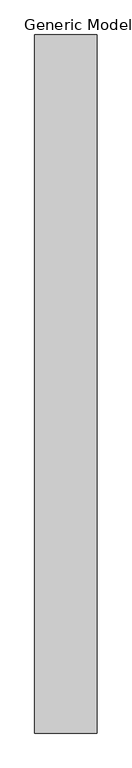
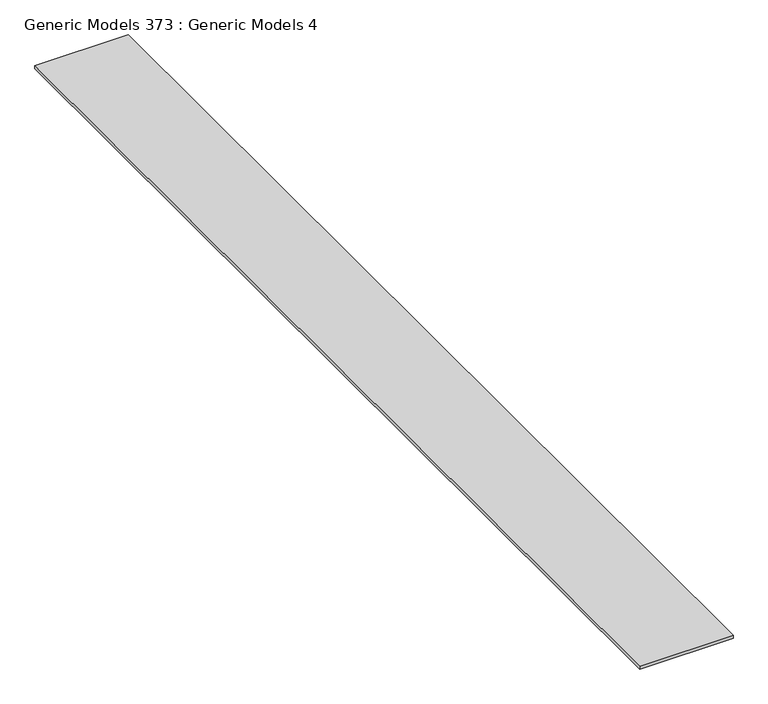
"""IFC4 building model written with IfcOpenShell, lengths in millimetres: proxy geometry, Generic Models 373 : Generic Models 4."""

from ifc_helpers import new_model, si_unit, frame, origin, place, context, project, spatial, polyline, outline, extrude, source, transform, mapped, element, save


def generic_models_373_generic_models_4_3e0b37f2(model_context):
    return source(origin(), model_context, "Body", "SweptSolid", [
        extrude(outline(polyline([(-6356.5236296, -6864.9230338), (-6928.2116813, -6864.9230338), (-6928.2116813, -464.1230338), (-6356.5236296, -464.1230338), (-6356.5236296, -6864.9230338)])), frame((0.0, 0.0, 129006.4087534), z_axis=(0.0, 0.0, 1.0), x_axis=(1.0, 0.0, 0.0)), (0.0, 0.0, 1.0), 18.9872466),
    ])


if __name__ == "__main__":
    model = new_model("IFC4")
    model_context = context("Model", 3, world=origin())
    ifc_project = project(units=[si_unit("LENGTHUNIT", "METRE", prefix="MILLI")], contexts=[model_context])
    site = spatial("IfcSite", under=ifc_project)
    building = spatial("IfcBuilding", under=site)
    placement = place(None, origin())
    generic_models_373_generic_models_4_shape = generic_models_373_generic_models_4_3e0b37f2(model_context)
    element("IfcBuildingElementProxy", 1, Name="Generic Models 373 : Generic Models 4", ObjectType="Generic Models 373 : Generic Models 4", at=placement, inside=building, context=model_context, shape_type="MappedRepresentation", body=[
        mapped(generic_models_373_generic_models_4_shape, transform((0.0, 0.0, 0.0), x_axis=(1.0, 0.0, 0.0), y_axis=(0.0, 1.0, 0.0), z_axis=(0.0, 0.0, 1.0))),
    ])
    save(model, "model.ifc")

# Revit data of these elements
# Element 1 (IfcBuildingElementProxy, "Generic Models 373 : Generic Models 4")
#   Materials on its faces: "_HARDWOOD VENEER PLYWOOD (GRADE B, OR BETTER) - MATCH SOLID TRIM SPECIES"
# Materials
#   "_HARDWOOD VENEER PLYWOOD (GRADE B, OR BETTER) - MATCH SOLID TRIM SPECIES": class "Generic", colour RGB 177 130 114, transparency 0, Cost = 0
